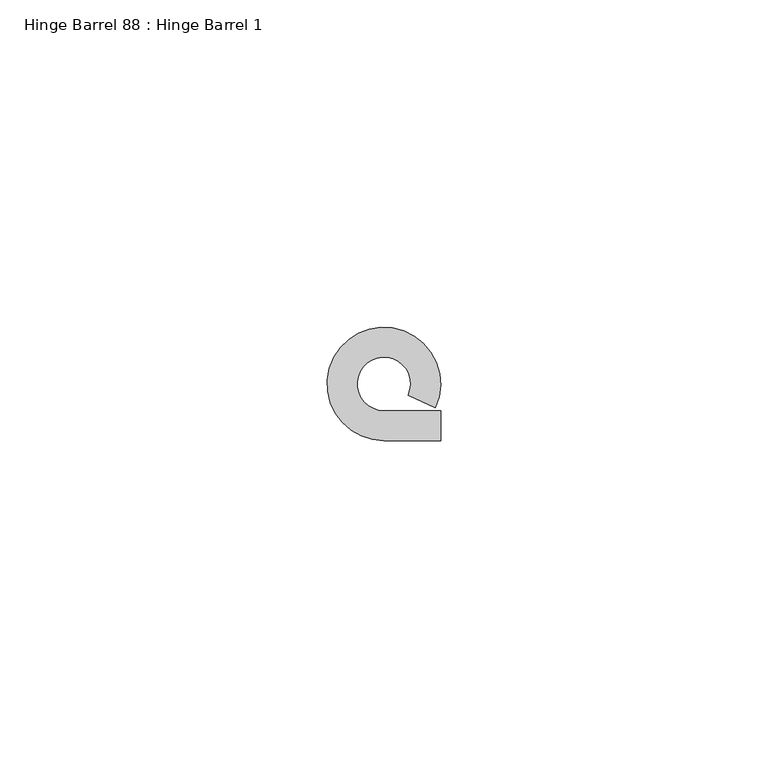
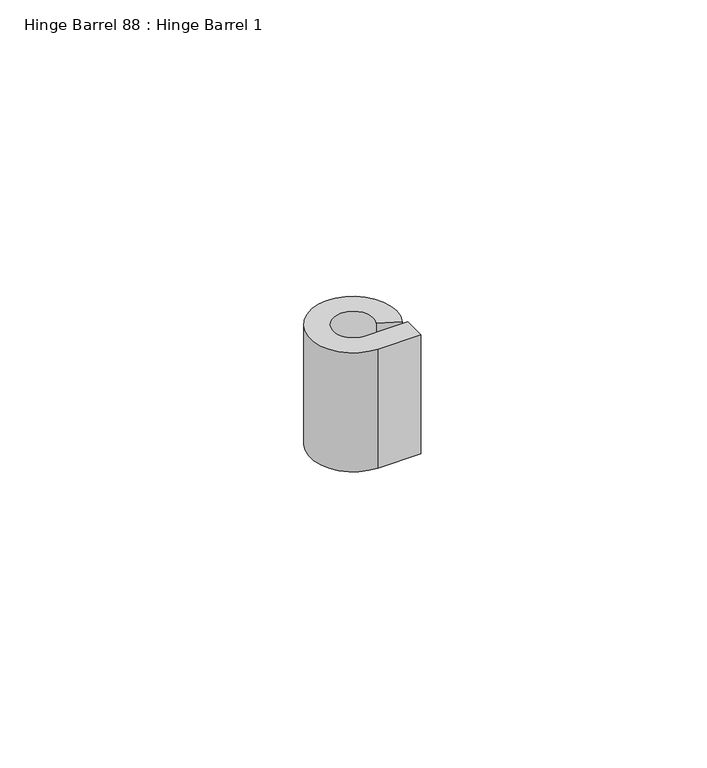
"""IFC4 building model written with IfcOpenShell, lengths in millimetres: proxy geometry, Hinge Barrel 88 : Hinge Barrel 1."""

from ifc_helpers import new_model, si_unit, point, frame, frame_2d, origin, place, context, project, spatial, polyline, circle_curve, trimmed, segment, composite_curve, outline, extrude, source, transform, mapped, element, save


def hinge_barrel_88_hinge_barrel_1_5bbaa909(model_context):
    return source(origin(), model_context, "Body", "SweptSolid", [
        extrude(outline(composite_curve([segment(polyline([(587323.2214739, -531780.6943841), (587327.7934739, -531780.6943841), (587327.7934739, -531785.2584466), (587319.1320739, -531785.2584466)]), True, "CONTINUOUS"), segment(trimmed(circle_curve(frame_2d((587319.1320739, -531776.6049841)), 8.6534625), [point((587319.1320739, -531785.2584466))], [point((587326.986084, -531780.2377433))], False, "CARTESIAN"), True, "CONTINUOUS"), segment(polyline([(587326.986084, -531780.2377433), (587322.8436736, -531778.321731)]), True, "CONTINUOUS"), segment(trimmed(circle_curve(frame_2d((587319.1320739, -531776.6049841)), 4.0894), [point((587322.8436736, -531778.321731))], [point((587319.1320739, -531780.6943841))], True, "CARTESIAN"), True, "CONTINUOUS"), segment(polyline([(587319.1320739, -531780.6943841), (587323.2214739, -531780.6943841)]), True, "CONTINUOUS")], self_intersect=False)), frame((0.0, 0.0, 1225.55), z_axis=(0.0, 0.0, 1.0), x_axis=(1.0, 0.0, 0.0)), (0.0, 0.0, 1.0), 25.4),
    ])


if __name__ == "__main__":
    model = new_model("IFC4")
    model_context = context("Model", 3, world=origin())
    ifc_project = project(units=[si_unit("LENGTHUNIT", "METRE", prefix="MILLI")], contexts=[model_context])
    site = spatial("IfcSite", under=ifc_project)
    building = spatial("IfcBuilding", under=site)
    placement = place(None, origin())
    hinge_barrel_88_hinge_barrel_1_shape = hinge_barrel_88_hinge_barrel_1_5bbaa909(model_context)
    element("IfcBuildingElementProxy", 1, Name="Hinge Barrel 88 : Hinge Barrel 1", ObjectType="Hinge Barrel 88 : Hinge Barrel 1", at=placement, inside=building, context=model_context, shape_type="MappedRepresentation", body=[
        mapped(hinge_barrel_88_hinge_barrel_1_shape, transform((0.0, 0.0, 0.0), x_axis=(1.0, 0.0, 0.0), y_axis=(0.0, 1.0, 0.0), z_axis=(0.0, 0.0, 1.0))),
    ])
    save(model, "model.ifc")

# Revit data of these elements
# Element 1 (IfcBuildingElementProxy, "Hinge Barrel 88 : Hinge Barrel 1")
#   Materials on its faces: "6\"X6\" WELD-ON STL BUTT HINGE"
# Materials
#   "6\"X6\" WELD-ON STL BUTT HINGE": class "Metal", colour RGB 189 187 185, transparency 0, Description = "Carbon steel", Cost = 0
